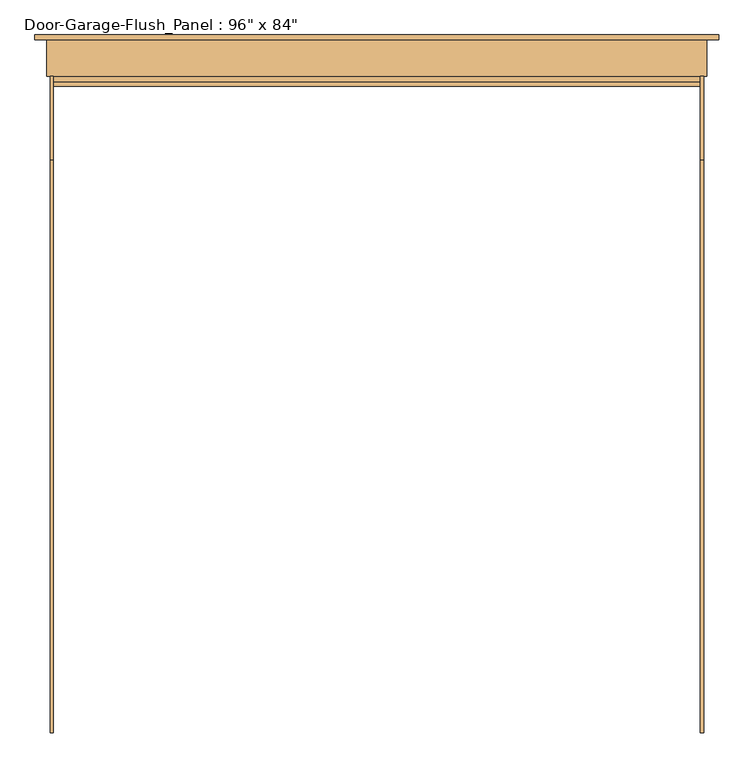
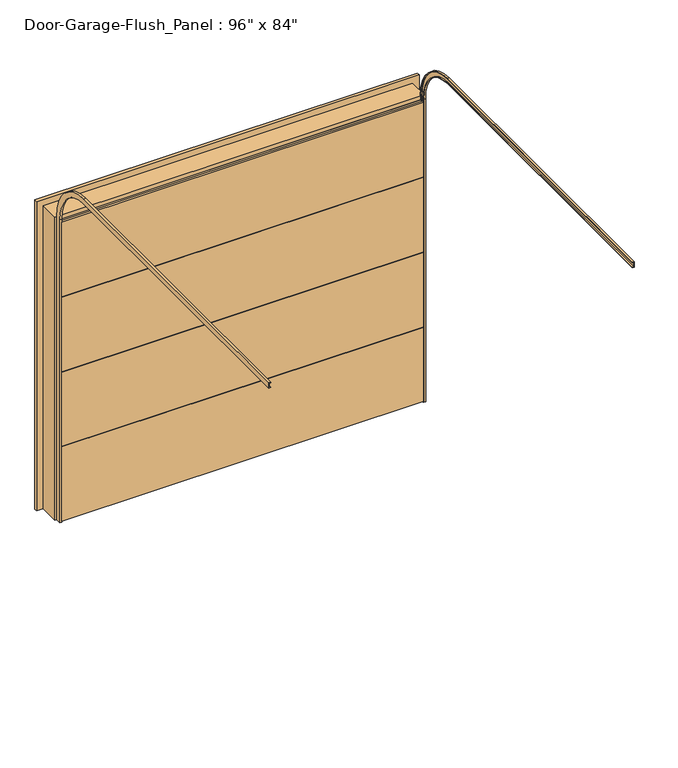
"""IFC4 building model written with IfcOpenShell, lengths in millimetres: door geometry."""

from ifc_helpers import new_model, si_unit, frame, origin, place, context, project, spatial, polyline, circle_curve, outline, extrude, source, transform, mapped, element, save
from ifc_brep_helpers import plane_surface, cylinder_surface, revolved_surface, advanced_brep


def door_bf818a00(model_context):
    return source(origin(), model_context, "Body", "SolidModel", [
        extrude(outline(polyline([(-93.6625, 2136.775), (-93.6625, 2130.425), (-71.4375, 2130.425), (-71.4375, 1600.2), (-87.3125, 1600.2), (-87.3125, 1606.55), (-109.5375, 1606.55), (-109.5375, 2136.775), (-93.6625, 2136.775)])), frame((-1219.2, 0.0, 0.0), z_axis=(1.0, 0.0, 0.0), x_axis=(0.0, 1.0, 0.0)), (0.0, 0.0, 1.0), 2438.4),
        extrude(outline(polyline([(-93.6625, 1603.375), (-93.6625, 1597.025), (-71.4375, 1597.025), (-71.4375, 1066.8), (-87.3125, 1066.8), (-87.3125, 1073.15), (-109.5375, 1073.15), (-109.5375, 1603.375), (-93.6625, 1603.375)])), frame((-1219.2, 0.0, 0.0), z_axis=(1.0, 0.0, 0.0), x_axis=(0.0, 1.0, 0.0)), (0.0, 0.0, 1.0), 2438.4),
        extrude(outline(polyline([(-93.6625, 1069.975), (-93.6625, 1063.625), (-71.4375, 1063.625), (-71.4375, 533.4), (-87.3125, 533.4), (-87.3125, 539.75), (-109.5375, 539.75), (-109.5375, 1069.975), (-93.6625, 1069.975)])), frame((-1219.2, 0.0, 0.0), z_axis=(1.0, 0.0, 0.0), x_axis=(0.0, 1.0, 0.0)), (0.0, 0.0, 1.0), 2438.4),
        extrude(outline(polyline([(-93.6625, 536.575), (-93.6625, 530.225), (-71.4375, 530.225), (-71.4375, 0.0), (-87.3125, 0.0), (-87.3125, 6.35), (-109.5375, 6.35), (-109.5375, 536.575), (-93.6625, 536.575)])), frame((-1219.2, 0.0, 0.0), z_axis=(1.0, 0.0, 0.0), x_axis=(0.0, 1.0, 0.0)), (0.0, 0.0, 1.0), 2438.4),
        advanced_brep(
        [(1231.9, -2547.9375, 2438.4), (1231.9, -2547.9375, 2476.5), (1219.2, -2547.9375, 2476.5), (1219.2, -2547.9375, 2473.325), (1228.725, -2547.9375, 2473.325), (1228.725, -2547.9375, 2441.575), (1219.2, -2547.9375, 2441.575), (1219.2, -2547.9375, 2438.4), (1231.9, -388.9375, 2438.4), (1231.9, -109.5375, 2159.0), (1231.9, -109.5375, 0.0), (1231.9, -71.4375, 0.0), (1231.9, -71.4375, 2159.0), (1231.9, -388.9375, 2476.5), (1219.2, -388.9375, 2476.5), (1219.2, -71.4375, 2159.0), (1219.2, -71.4375, 0.0), (1219.2, -74.6125, 0.0), (1219.2, -74.6125, 2159.0), (1219.2, -388.9375, 2473.325), (1228.725, -388.9375, 2473.325), (1228.725, -74.6125, 2159.0), (1228.725, -74.6125, 0.0), (1228.725, -106.3625, 0.0), (1228.725, -106.3625, 2159.0), (1228.725, -388.9375, 2441.575), (1219.2, -388.9375, 2441.575), (1219.2, -106.3625, 2159.0), (1219.2, -106.3625, 0.0), (1219.2, -109.5375, 0.0), (1219.2, -109.5375, 2159.0), (1219.2, -388.9375, 2438.4)],
        [
            (0, 1),
            (1, 2),
            (2, 3),
            (3, 4),
            (4, 5),
            (5, 6),
            (6, 7),
            (7, 0),
            (0, 8),
            (8, 9, circle_curve(frame((1231.9, -388.9375, 2159.0), z_axis=(-1.0, 0.0, 0.0), x_axis=(0.0, 0.0, 1.0)), 279.4)),
            (9, 10),
            (10, 11),
            (11, 12),
            (12, 13, circle_curve(frame((1231.9, -388.9375, 2159.0), z_axis=(1.0, 0.0, 0.0), x_axis=(0.0, 0.0, 1.0)), 317.5)),
            (13, 1),
            (13, 14),
            (14, 2),
            (14, 15, circle_curve(frame((1219.2, -388.9375, 2159.0), z_axis=(-1.0, 0.0, 0.0), x_axis=(0.0, 0.0, 1.0)), 317.5)),
            (15, 16),
            (16, 17),
            (17, 18),
            (18, 19, circle_curve(frame((1219.2, -388.9375, 2159.0), z_axis=(1.0, 0.0, 0.0), x_axis=(0.0, 0.0, 1.0)), 314.325)),
            (19, 3),
            (19, 20),
            (20, 4),
            (20, 21, circle_curve(frame((1228.725, -388.9375, 2159.0), z_axis=(-1.0, 0.0, 0.0), x_axis=(0.0, 0.0, 1.0)), 314.325)),
            (21, 22),
            (22, 23),
            (23, 24),
            (24, 25, circle_curve(frame((1228.725, -388.9375, 2159.0), z_axis=(1.0, 0.0, 0.0), x_axis=(0.0, 0.0, 1.0)), 282.575)),
            (25, 5),
            (25, 26),
            (26, 6),
            (26, 27, circle_curve(frame((1219.2, -388.9375, 2159.0), z_axis=(-1.0, 0.0, 0.0), x_axis=(0.0, 0.0, 1.0)), 282.575)),
            (27, 28),
            (28, 29),
            (29, 30),
            (30, 31, circle_curve(frame((1219.2, -388.9375, 2159.0), z_axis=(1.0, 0.0, 0.0), x_axis=(0.0, 0.0, 1.0)), 279.4)),
            (31, 7),
            (31, 8),
            (12, 15),
            (18, 21),
            (24, 27),
            (30, 9),
            (10, 29),
            (28, 23),
            (22, 17),
            (16, 11),
        ],
        [
            plane_surface(frame((0.0, -2547.9375, 2438.4), z_axis=(0.0, -1.0, 0.0), x_axis=(1.0, 0.0, 0.0))),
            plane_surface(frame((1231.9, -2547.9375, 2438.4), z_axis=(1.0, 0.0, 0.0), x_axis=(0.0, 1.0, 0.0))),
            plane_surface(frame((1231.9, -2547.9375, 2476.5), z_axis=(0.0, 0.0, 1.0), x_axis=(0.0, 1.0, 0.0))),
            plane_surface(frame((1219.2, -2547.9375, 2476.5), z_axis=(-1.0, 0.0, 0.0), x_axis=(0.0, 1.0, 0.0))),
            plane_surface(frame((1219.2, -2547.9375, 2473.325), z_axis=(0.0, 0.0, -1.0), x_axis=(0.0, 1.0, 0.0))),
            plane_surface(frame((1228.725, -2547.9375, 2473.325), z_axis=(-1.0, 0.0, 0.0), x_axis=(0.0, 1.0, 0.0))),
            plane_surface(frame((1228.725, -2547.9375, 2441.575), z_axis=(0.0, 0.0, 1.0), x_axis=(0.0, 1.0, 0.0))),
            plane_surface(frame((1219.2, -2547.9375, 2441.575), z_axis=(-1.0, 0.0, 0.0), x_axis=(0.0, 1.0, 0.0))),
            plane_surface(frame((1219.2, -2547.9375, 2438.4), z_axis=(0.0, 0.0, -1.0), x_axis=(0.0, 1.0, 0.0))),
            cylinder_surface(frame((0.0, -388.9375, 2159.0), z_axis=(-1.0, 0.0, 0.0), x_axis=(0.0, 0.0, 1.0)), 317.5),
            revolved_surface(polyline([(1219.2, -388.9375, 2473.325), (1228.725, -388.9375, 2473.325)]), (0.0, -388.9375, 2159.0), (-1.0, 0.0, 0.0)),
            cylinder_surface(frame((0.0, -388.9375, 2159.0), z_axis=(-1.0, 0.0, 0.0), x_axis=(0.0, 0.0, 1.0)), 282.575),
            revolved_surface(polyline([(1219.2, -388.9375, 2438.4), (1231.9, -388.9375, 2438.4)]), (0.0, -388.9375, 2159.0), (-1.0, 0.0, 0.0)),
            plane_surface(frame((0.0, -109.5375, 0.0), z_axis=(0.0, 0.0, -1.0), x_axis=(1.0, 0.0, 0.0))),
            plane_surface(frame((1231.9, -71.4375, 2159.0), z_axis=(0.0, 1.0, 0.0), x_axis=(0.0, 0.0, -1.0))),
            plane_surface(frame((1219.2, -74.6125, 2159.0), z_axis=(0.0, -1.0, 0.0), x_axis=(0.0, 0.0, -1.0))),
            plane_surface(frame((1228.725, -106.3625, 2159.0), z_axis=(0.0, 1.0, 0.0), x_axis=(0.0, 0.0, -1.0))),
            plane_surface(frame((1219.2, -109.5375, 2159.0), z_axis=(0.0, -1.0, 0.0), x_axis=(0.0, 0.0, -1.0))),
        ],
        [
            (0, [[1, 2, 3, 4, 5, 6, 7, 8]]),
            (1, [[-1, 9, 10, 11, 12, 13, 14, 15]]),
            (2, [[-2, -15, 16, 17]]),
            (3, [[-3, -17, 18, 19, 20, 21, 22, 23]]),
            (4, [[-4, -23, 24, 25]]),
            (5, [[-5, -25, 26, 27, 28, 29, 30, 31]]),
            (6, [[-6, -31, 32, 33]]),
            (7, [[-7, -33, 34, 35, 36, 37, 38, 39]]),
            (8, [[-8, -39, 40, -9]]),
            (9, [[-18, -16, -14, 41]]),
            (10, [[-26, -24, -22, 42]]),
            (11, [[-34, -32, -30, 43]]),
            (12, [[-10, -40, -38, 44]]),
            (13, [[45, -36, 46, -28, 47, -20, 48, -12]]),
            (14, [[-41, -13, -48, -19]]),
            (15, [[-42, -21, -47, -27]]),
            (16, [[-43, -29, -46, -35]]),
            (17, [[-44, -37, -45, -11]]),
        ],
    ),
        advanced_brep(
        [(-1231.9, -2547.9375, 2438.4), (-1219.2, -2547.9375, 2438.4), (-1219.2, -2547.9375, 2441.575), (-1228.725, -2547.9375, 2441.575), (-1228.725, -2547.9375, 2473.325), (-1219.2, -2547.9375, 2473.325), (-1219.2, -2547.9375, 2476.5), (-1231.9, -2547.9375, 2476.5), (-1231.9, -388.9375, 2438.4), (-1219.2, -388.9375, 2438.4), (-1219.2, -109.5375, 2159.0), (-1219.2, -109.5375, 0.0), (-1219.2, -106.3625, 0.0), (-1219.2, -106.3625, 2159.0), (-1219.2, -388.9375, 2441.575), (-1228.725, -388.9375, 2441.575), (-1228.725, -106.3625, 2159.0), (-1228.725, -106.3625, 0.0), (-1228.725, -74.6125, 0.0), (-1228.725, -74.6125, 2159.0), (-1228.725, -388.9375, 2473.325), (-1219.2, -388.9375, 2473.325), (-1219.2, -74.6125, 2159.0), (-1219.2, -74.6125, 0.0), (-1219.2, -71.4375, 0.0), (-1219.2, -71.4375, 2159.0), (-1219.2, -388.9375, 2476.5), (-1231.9, -388.9375, 2476.5), (-1231.9, -71.4375, 2159.0), (-1231.9, -71.4375, 0.0), (-1231.9, -109.5375, 0.0), (-1231.9, -109.5375, 2159.0)],
        [
            (0, 1),
            (1, 2),
            (2, 3),
            (3, 4),
            (4, 5),
            (5, 6),
            (6, 7),
            (7, 0),
            (0, 8),
            (8, 9),
            (9, 1),
            (9, 10, circle_curve(frame((-1219.2, -388.9375, 2159.0), z_axis=(-1.0, 0.0, 0.0), x_axis=(0.0, 0.0, 1.0)), 279.4)),
            (10, 11),
            (11, 12),
            (12, 13),
            (13, 14, circle_curve(frame((-1219.2, -388.9375, 2159.0), z_axis=(1.0, 0.0, 0.0), x_axis=(0.0, 0.0, 1.0)), 282.575)),
            (14, 2),
            (14, 15),
            (15, 3),
            (15, 16, circle_curve(frame((-1228.725, -388.9375, 2159.0), z_axis=(-1.0, 0.0, 0.0), x_axis=(0.0, 0.0, 1.0)), 282.575)),
            (16, 17),
            (17, 18),
            (18, 19),
            (19, 20, circle_curve(frame((-1228.725, -388.9375, 2159.0), z_axis=(1.0, 0.0, 0.0), x_axis=(0.0, 0.0, 1.0)), 314.325)),
            (20, 4),
            (20, 21),
            (21, 5),
            (21, 22, circle_curve(frame((-1219.2, -388.9375, 2159.0), z_axis=(-1.0, 0.0, 0.0), x_axis=(0.0, 0.0, 1.0)), 314.325)),
            (22, 23),
            (23, 24),
            (24, 25),
            (25, 26, circle_curve(frame((-1219.2, -388.9375, 2159.0), z_axis=(1.0, 0.0, 0.0), x_axis=(0.0, 0.0, 1.0)), 317.5)),
            (26, 6),
            (26, 27),
            (27, 7),
            (27, 28, circle_curve(frame((-1231.9, -388.9375, 2159.0), z_axis=(-1.0, 0.0, 0.0), x_axis=(0.0, 0.0, 1.0)), 317.5)),
            (28, 29),
            (29, 30),
            (30, 31),
            (31, 8, circle_curve(frame((-1231.9, -388.9375, 2159.0), z_axis=(1.0, 0.0, 0.0), x_axis=(0.0, 0.0, 1.0)), 279.4)),
            (31, 10),
            (13, 16),
            (19, 22),
            (25, 28),
            (29, 24),
            (23, 18),
            (17, 12),
            (11, 30),
        ],
        [
            plane_surface(frame((0.0, -2547.9375, 2438.4), z_axis=(0.0, -1.0, 0.0), x_axis=(1.0, 0.0, 0.0))),
            plane_surface(frame((-1231.9, -2547.9375, 2438.4), z_axis=(0.0, 0.0, -1.0), x_axis=(0.0, 1.0, 0.0))),
            plane_surface(frame((-1219.2, -2547.9375, 2438.4), z_axis=(1.0, 0.0, 0.0), x_axis=(0.0, 1.0, 0.0))),
            plane_surface(frame((-1219.2, -2547.9375, 2441.575), z_axis=(0.0, 0.0, 1.0), x_axis=(0.0, 1.0, 0.0))),
            plane_surface(frame((-1228.725, -2547.9375, 2441.575), z_axis=(1.0, 0.0, 0.0), x_axis=(0.0, 1.0, 0.0))),
            plane_surface(frame((-1228.725, -2547.9375, 2473.325), z_axis=(0.0, 0.0, -1.0), x_axis=(0.0, 1.0, 0.0))),
            plane_surface(frame((-1219.2, -2547.9375, 2473.325), z_axis=(1.0, 0.0, 0.0), x_axis=(0.0, 1.0, 0.0))),
            plane_surface(frame((-1219.2, -2547.9375, 2476.5), z_axis=(0.0, 0.0, 1.0), x_axis=(0.0, 1.0, 0.0))),
            plane_surface(frame((-1231.9, -2547.9375, 2476.5), z_axis=(-1.0, 0.0, 0.0), x_axis=(0.0, 1.0, 0.0))),
            revolved_surface(polyline([(-1231.9, -388.9375, 2438.4), (-1219.2, -388.9375, 2438.4)]), (0.0, -388.9375, 2159.0), (-1.0, 0.0, 0.0)),
            cylinder_surface(frame((0.0, -388.9375, 2159.0), z_axis=(-1.0, 0.0, 0.0), x_axis=(0.0, 0.0, 1.0)), 282.575),
            revolved_surface(polyline([(-1228.725, -388.9375, 2473.325), (-1219.2, -388.9375, 2473.325)]), (0.0, -388.9375, 2159.0), (-1.0, 0.0, 0.0)),
            cylinder_surface(frame((0.0, -388.9375, 2159.0), z_axis=(-1.0, 0.0, 0.0), x_axis=(0.0, 0.0, 1.0)), 317.5),
            plane_surface(frame((0.0, -109.5375, 0.0), z_axis=(0.0, 0.0, -1.0), x_axis=(1.0, 0.0, 0.0))),
            plane_surface(frame((-1231.9, -109.5375, 2159.0), z_axis=(0.0, -1.0, 0.0), x_axis=(0.0, 0.0, -1.0))),
            plane_surface(frame((-1219.2, -106.3625, 2159.0), z_axis=(0.0, 1.0, 0.0), x_axis=(0.0, 0.0, -1.0))),
            plane_surface(frame((-1228.725, -74.6125, 2159.0), z_axis=(0.0, -1.0, 0.0), x_axis=(0.0, 0.0, -1.0))),
            plane_surface(frame((-1219.2, -71.4375, 2159.0), z_axis=(0.0, 1.0, 0.0), x_axis=(0.0, 0.0, -1.0))),
        ],
        [
            (0, [[1, 2, 3, 4, 5, 6, 7, 8]]),
            (1, [[-1, 9, 10, 11]]),
            (2, [[-2, -11, 12, 13, 14, 15, 16, 17]]),
            (3, [[-3, -17, 18, 19]]),
            (4, [[-4, -19, 20, 21, 22, 23, 24, 25]]),
            (5, [[-5, -25, 26, 27]]),
            (6, [[-6, -27, 28, 29, 30, 31, 32, 33]]),
            (7, [[-7, -33, 34, 35]]),
            (8, [[-8, -35, 36, 37, 38, 39, 40, -9]]),
            (9, [[-12, -10, -40, 41]]),
            (10, [[-20, -18, -16, 42]]),
            (11, [[-28, -26, -24, 43]]),
            (12, [[-36, -34, -32, 44]]),
            (13, [[-38, 45, -30, 46, -22, 47, -14, 48]]),
            (14, [[-41, -39, -48, -13]]),
            (15, [[-42, -15, -47, -21]]),
            (16, [[-43, -23, -46, -29]]),
            (17, [[-44, -31, -45, -37]]),
        ],
    ),
        extrude(outline(polyline([(0.0, 1219.2), (0.0, 1244.6), (2159.0, 1244.6), (2159.0, -1244.6), (0.0, -1244.6), (0.0, -1219.2), (2133.6, -1219.2), (2133.6, 1219.2), (0.0, 1219.2)])), frame((0.0, -71.4375, 0.0), z_axis=(0.0, 1.0, 0.0), x_axis=(0.0, 0.0, 1.0)), (0.0, 0.0, 1.0), 136.525),
        extrude(outline(polyline([(0.0, 1225.55), (0.0, 1289.05), (2203.45, 1289.05), (2203.45, -1289.05), (0.0, -1289.05), (0.0, -1225.55), (2139.95, -1225.55), (2139.95, 1225.55), (0.0, 1225.55)])), frame((0.0, 65.0875, 0.0), z_axis=(0.0, 1.0, 0.0), x_axis=(0.0, 0.0, 1.0)), (0.0, 0.0, 1.0), 19.05),
    ])


if __name__ == "__main__":
    model = new_model("IFC4")
    model_context = context("Model", 3, world=origin())
    ifc_project = project(units=[si_unit("LENGTHUNIT", "METRE", prefix="MILLI")], contexts=[model_context])
    site = spatial("IfcSite", under=ifc_project)
    building = spatial("IfcBuilding", under=site)
    placement = place(None, origin())
    door_shape = door_bf818a00(model_context)
    element("IfcDoor", 1, ObjectType="Door-Garage-Flush_Panel : 96\" x 84\"", at=placement, inside=building, context=model_context, shape_type="MappedRepresentation", body=[
        mapped(door_shape, transform((0.0, 0.0, 0.0), x_axis=(1.0, 0.0, 0.0), y_axis=(0.0, 1.0, 0.0), z_axis=(0.0, 0.0, 1.0))),
    ])
    save(model, "model.ifc")

# Revit data of these elements
# Type "Door-Garage-Flush_Panel : 96\" x 84\""
#   Type Mark = "49"
#   Assembly Code = "B2030400"
#   Analytic Construction = "Wooden"
#   Thickness = 0' - 1 1/2"
#   Thermal Resistance (R) = 0.455703 (m²·K)/W
#   Rough Width = 8' - 2"
#   Rough Height = 7' - 1"
#   Panel Height = 1' - 9"
#   Height = 7' - 0"
#   Width = 8' - 0"
#   Heat Transfer Coefficient (U) = 2.19465 W/(m²·K)
#   Function = 1
#   Exterior Trim [instance default] = yes
#   Trim Material = Cherry
#   Panel Material = Cherry
#   Frame Material = Cherry
#   Visual Light Transmittance = 0
#   Solar Heat Gain Coefficient = 0
#   Wall Closure = (empty or 0)
# Element 1 (IfcDoor, "Door-Garage-Flush_Panel : 96\" x 84\"")
#   Materials on its faces: "Cherry"
# Materials
#   "Cherry": class "Wood", colour RGB 226 177 128, transparency 0, Description = "Prunus Serotina", Cost = 0
